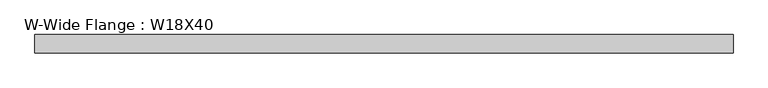
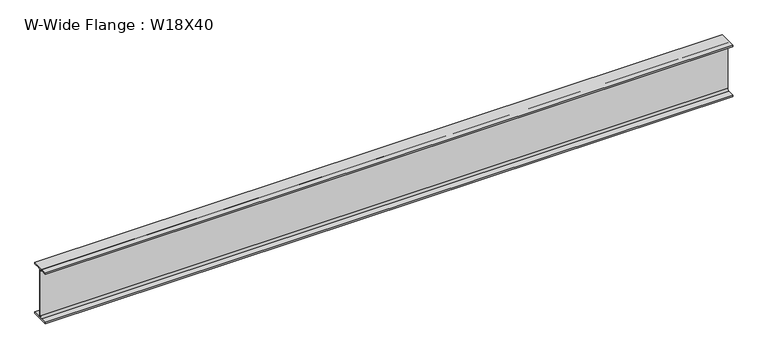
"""IFC4 building model written with IfcOpenShell, lengths in millimetres: beam geometry, W-Wide Flange : W18X40."""

from ifc_helpers import new_model, si_unit, point, frame, frame_2d, origin, place, context, project, spatial, polyline, circle_curve, trimmed, segment, composite_curve, outline, extrude, source, transform, mapped, element, save


def w_wide_flange_w18x40_9d12e89c(model_context):
    return source(origin(), model_context, "Body", "SweptSolid", [
        extrude(outline(composite_curve([segment(polyline([(76.454, -213.995), (76.454, -227.33), (-76.454, -227.33), (-76.454, -213.995), (-20.828, -213.995)]), True, "CONTINUOUS"), segment(trimmed(circle_curve(frame_2d((-20.828, -197.1675)), 16.8275), [point((-20.828, -213.995))], [point((-4.0005, -197.1675))], True, "CARTESIAN"), True, "CONTINUOUS"), segment(polyline([(-4.0005, -197.1675), (-4.0005, 197.1675)]), True, "CONTINUOUS"), segment(trimmed(circle_curve(frame_2d((-20.828, 197.1675)), 16.8275), [point((-4.0005, 197.1675))], [point((-20.828, 213.995))], True, "CARTESIAN"), True, "CONTINUOUS"), segment(polyline([(-20.828, 213.995), (-76.454, 213.995), (-76.454, 227.33), (76.454, 227.33), (76.454, 213.995), (20.828, 213.995)]), True, "CONTINUOUS"), segment(trimmed(circle_curve(frame_2d((20.828, 197.1675)), 16.8275), [point((20.828, 213.995))], [point((4.0005, 197.1675))], True, "CARTESIAN"), True, "CONTINUOUS"), segment(polyline([(4.0005, 197.1675), (4.0005, -197.1675)]), True, "CONTINUOUS"), segment(trimmed(circle_curve(frame_2d((20.828, -197.1675)), 16.8275), [point((4.0005, -197.1675))], [point((20.828, -213.995))], True, "CARTESIAN"), True, "CONTINUOUS"), segment(polyline([(20.828, -213.995), (76.454, -213.995)]), True, "CONTINUOUS")], self_intersect=False)), frame((-2876.55, 0.0, 0.0), z_axis=(1.0, 0.0, 0.0), x_axis=(0.0, 1.0, 0.0)), (0.0, 0.0, 1.0), 5758.18),
    ])


if __name__ == "__main__":
    model = new_model("IFC4")
    model_context = context("Model", 3, world=origin())
    ifc_project = project(units=[si_unit("LENGTHUNIT", "METRE", prefix="MILLI")], contexts=[model_context])
    site = spatial("IfcSite", under=ifc_project)
    building = spatial("IfcBuilding", under=site)
    placement = place(None, origin())
    w_wide_flange_w18x40_shape = w_wide_flange_w18x40_9d12e89c(model_context)
    element("IfcBeam", 1, ObjectType="W-Wide Flange : W18X40", at=placement, inside=building, context=model_context, shape_type="MappedRepresentation", body=[
        mapped(w_wide_flange_w18x40_shape, transform((0.0, 0.0, 0.0), x_axis=(1.0, 0.0, 0.0), y_axis=(0.0, 1.0, 0.0), z_axis=(0.0, 0.0, 1.0))),
    ])
    save(model, "model.ifc")

# Revit data of these elements
# Type "W-Wide Flange : W18X40"
#   Assembly Code = "B10"
#   W = 40
#   Length [instance default] = 5' - 0"
#   bf = 0' - 6.02"
#   d = 1' - 5.9"
#   k = 0' - 1 3/16"
#   k2 = 0' - 0.6625"
#   tf = 0' - 0.525"
#   tw = 0' - 0.315"
#   A = 0.0819444 SF
#   Structural Material [instance default] = Steel ASTM A992
# Element 1 (IfcBeam, "W-Wide Flange : W18X40")
#   Materials on its faces: "Steel ASTM A992"
# Materials
#   "Steel ASTM A992": class "Metal", colour RGB 199 199 199, transparency 0, Description = "Structural steel 50ksi", Cost = 0
